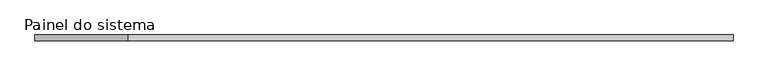
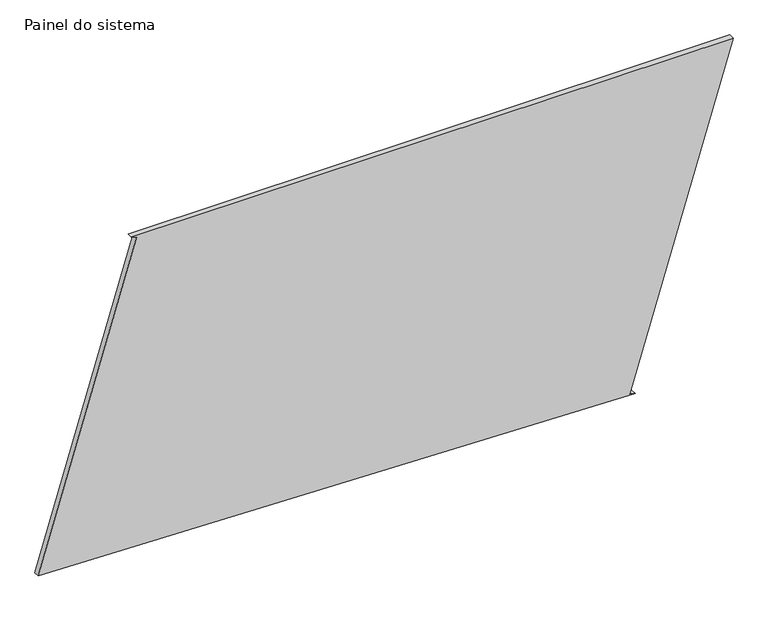
"""IFC4 building model written with IfcOpenShell, lengths in millimetres: plate geometry, Painel do sistema : Envidraçado."""

from ifc_helpers import new_model, si_unit, frame, origin, place, context, project, spatial, polyline, outline, extrude, source, transform, mapped, element, save


def painel_do_sistema_c67f19d5(model_context):
    return source(origin(), model_context, "Body", "SweptSolid", [
        extrude(outline(polyline([(0.0, 1103.8681374), (7.2712141, 1079.9489098), (1512.2998163, 1537.4630646), (1512.2998163, -1125.2785882), (1505.0286022, -1101.3593606), (70.4313529, -1537.4630646), (0.0, 1103.8681374)])), frame((0.0, 24.5, 0.0), z_axis=(0.0, 1.0, 0.0), x_axis=(0.0, 0.0, 1.0)), (0.0, 0.0, 1.0), 25.0),
    ])


if __name__ == "__main__":
    model = new_model("IFC4")
    model_context = context("Model", 3, world=origin())
    ifc_project = project(units=[si_unit("LENGTHUNIT", "METRE", prefix="MILLI")], contexts=[model_context])
    site = spatial("IfcSite", under=ifc_project)
    building = spatial("IfcBuilding", under=site)
    placement = place(None, origin())
    painel_do_sistema_shape = painel_do_sistema_c67f19d5(model_context)
    element("IfcPlate", 1, ObjectType="Painel do sistema : Envidraçado", at=placement, inside=building, context=model_context, shape_type="MappedRepresentation", body=[
        mapped(painel_do_sistema_shape, transform((0.0, 0.0, 0.0), x_axis=(1.0, 0.0, 0.0), y_axis=(0.0, 1.0, 0.0), z_axis=(0.0, 0.0, 1.0))),
    ])
    save(model, "model.ifc")

# Revit data of these elements
# Type "Painel do sistema : Envidraçado"
#   Construction Type Id = "GSP4R"
#   Analytic Construction = "Vidraça única Pilkington 1/8 pol"
#   Visual Light Transmittance = 0.9
#   Solar Heat Gain Coefficient = 0.86
#   Heat Transfer Coefficient (U) = 6.7069 W/(m²·K)
# Element 1 (IfcPlate, "Painel do sistema : Envidraçado")
#   Materials on its faces: "Vidro"
# Materials
#   "Vidro": class "Vidro", colour RGB 0 128 192, transparency 0.9, Description = "Vidro de sílica", Cost = 0
